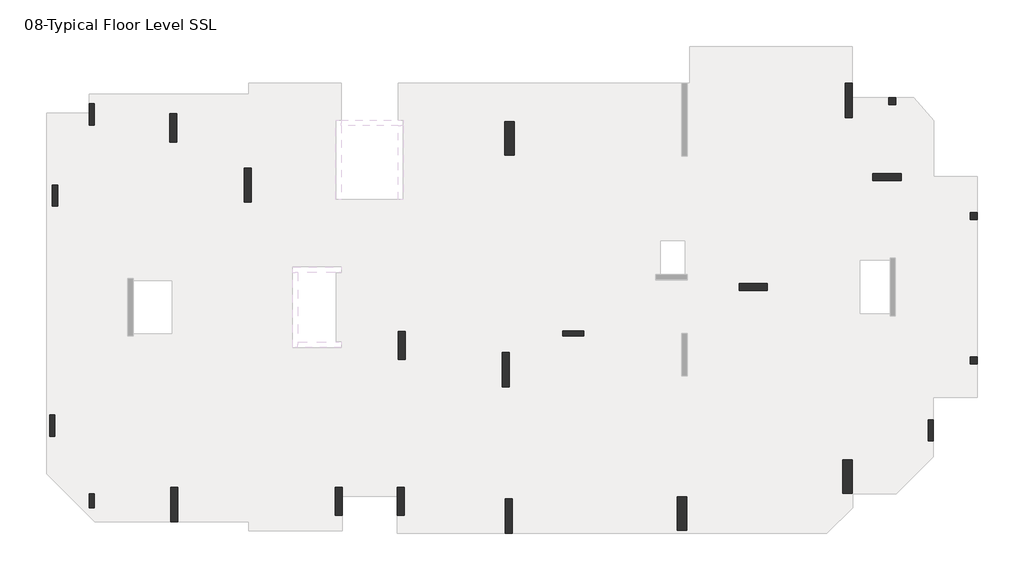
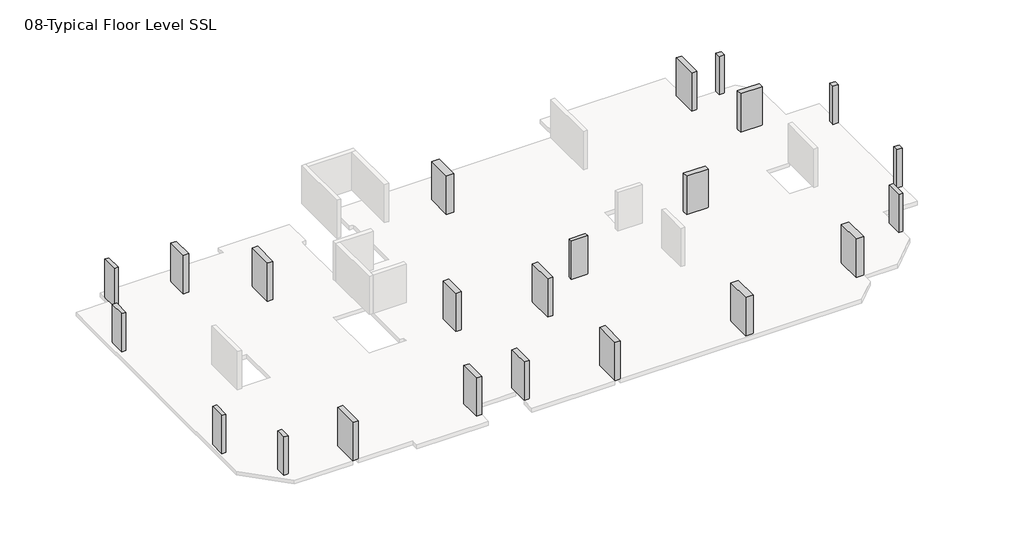
# One storey, part 2 of 2: 23 columns.
"""IFC4 building model written with IfcOpenShell, lengths in millimetres."""

from ifc_helpers import new_model, si_unit, origin, place, context, project, spatial, faceted_brep, element, save

model = new_model("IFC4")

# Units and contexts
model_context = context("Model", 3, world=origin())
ifc_project = project(units=[si_unit("LENGTHUNIT", "METRE", prefix="MILLI")], contexts=[model_context])

# Site, building, storey
site = spatial("IfcSite", under=ifc_project)
building = spatial("IfcBuilding", under=site)
storey = spatial("IfcBuildingStorey", under=building, Name="08-Typical Floor Level SSL", Elevation=18000.0)

# Columns
placement = place(None, origin())
element("IfcColumn", 1, ObjectType="M_Concrete-Rectangular-Column : C-1 (400 x 400mm)", at=placement, inside=storey, context=model_context, shape_type="Brep", body=[
    faceted_brep([(52549.9999998, 16712.0, 18000.0), (52549.9999998, 16312.0, 18000.0), (52149.9999998, 16312.0, 18000.0), (52149.9999998, 16712.0, 18000.0), (52549.9999998, 16712.0, 21000.0), (52549.9999998, 16312.0, 21000.0), (52549.9999998, 16312.0, 20700.0), (52549.9999998, 16712.0, 20700.0), (52149.9999998, 16312.0, 21000.0), (52149.9999998, 16312.0, 20700.0), (52149.9999998, 16712.0, 21000.0), (52149.9999998, 16712.0, 20700.0)], [[[0, 1, 2, 3]], [[4, 5, 6, 1, 0, 7]], [[5, 8, 9, 2, 1, 6]], [[8, 10, 11, 3, 2, 9]], [[10, 4, 7, 0, 3, 11]], [[4, 10, 8, 5]]]),
])
element("IfcColumn", 2, ObjectType="M_Concrete-Rectangular-Column : C-1 (400 x 400mm)", at=placement, inside=storey, context=model_context, shape_type="Brep", body=[
    faceted_brep([(47898.6337868, 23252.0, 18000.0), (47898.6337868, 22852.0, 18000.0), (47498.6337868, 22852.0, 18000.0), (47498.6337868, 23252.0, 18000.0), (47898.6337868, 23252.0, 21000.0), (47898.6337868, 22852.0, 21000.0), (47898.6337868, 22852.0, 20700.0), (47498.6337868, 22852.0, 21000.0), (47498.6337868, 22852.0, 20700.0), (47498.6337868, 23252.0, 21000.0)], [[[0, 1, 2, 3]], [[4, 5, 6, 1, 0]], [[5, 7, 8, 2, 1, 6]], [[7, 9, 3, 2, 8]], [[9, 4, 0, 3]], [[4, 9, 7, 5]]]),
])
element("IfcColumn", 3, ObjectType="M_Concrete-Rectangular-Column : C-1 (400 x 400mm)", at=placement, inside=storey, context=model_context, shape_type="Brep", body=[
    faceted_brep([(52549.9999998, 8504.0039609, 18000.0), (52549.9999998, 8104.0039609, 18000.0), (52149.9999998, 8104.0039609, 18000.0), (52149.9999998, 8504.0039609, 18000.0), (52549.9999998, 8504.0039609, 21000.0), (52549.9999998, 8104.0039609, 21000.0), (52549.9999998, 8104.0039609, 20700.0), (52549.9999998, 8504.0039609, 20700.0), (52149.9999998, 8104.0039609, 21000.0), (52149.9999998, 8104.0039609, 20700.0), (52149.9999998, 8504.0039609, 21000.0), (52149.9999998, 8504.0039609, 20700.0)], [[[0, 1, 2, 3]], [[4, 5, 6, 1, 0, 7]], [[5, 8, 9, 2, 1, 6]], [[8, 10, 11, 3, 2, 9]], [[10, 4, 7, 0, 3, 11]], [[4, 10, 8, 5]]]),
])
element("IfcColumn", 4, ObjectType="M_Concrete-Rectangular-Column : C-2 (300 x 800mm)", at=placement, inside=storey, context=model_context, shape_type="Brep", body=[
    faceted_brep([(2352.0, 728.0, 18000.0), (2352.0, -72.0, 18000.0), (2052.0, -72.0, 18000.0), (2052.0, 728.0, 18000.0), (2352.0, 728.0, 21000.0), (2352.0, -72.0, 21000.0), (2352.0, -72.0, 20700.0), (2352.0, 728.0, 20700.0), (2052.0, -72.0, 21000.0), (2052.0, -72.0, 20700.0), (2052.0, 728.0, 21000.0), (2052.0, 728.0, 20700.0)], [[[0, 1, 2, 3]], [[4, 5, 6, 1, 0, 7]], [[5, 8, 9, 2, 1, 6]], [[8, 10, 11, 3, 2, 9]], [[10, 4, 7, 0, 3, 11]], [[4, 10, 8, 5]]]),
])
element("IfcColumn", 5, ObjectType="M_Concrete-Rectangular-Column : C-3(300 x 1200mm)", at=placement, inside=storey, context=model_context, shape_type="Brep", body=[
    faceted_brep([(2352.0, 22908.0000656, 18000.0), (2352.0, 21708.0000656, 18000.0), (2052.0, 21708.0000656, 18000.0), (2052.0, 22908.0000656, 18000.0), (2352.0, 22908.0000656, 21000.0), (2352.0, 21708.0000656, 21000.0), (2352.0, 21708.0000656, 20700.0), (2352.0, 22908.0000656, 20700.0), (2052.0, 21708.0000656, 21000.0), (2052.0, 21708.0000656, 20700.0), (2052.0, 22380.0004589, 21000.0), (2052.0, 22908.0000656, 21000.0), (2052.0, 22908.0000656, 20700.0)], [[[0, 1, 2, 3]], [[4, 5, 6, 1, 0, 7]], [[5, 8, 9, 2, 1, 6]], [[8, 10, 11, 12, 3, 2, 9]], [[11, 4, 7, 0, 3, 12]], [[4, 11, 10, 8, 5]]]),
])
element("IfcColumn", 6, ObjectType="M_Concrete-Rectangular-Column : C-3(300 x 1200mm)", at=placement, inside=storey, context=model_context, shape_type="Brep", body=[
    faceted_brep([(257.9999999, 18288.0, 18000.0), (257.9999999, 17088.0, 18000.0), (-42.0000001, 17088.0, 18000.0), (-42.0000001, 18288.0, 18000.0), (257.9999999, 18288.0, 21000.0), (257.9999999, 17088.0, 21000.0), (257.9999999, 17088.0, 20700.0), (257.9999999, 18288.0, 20700.0), (-42.0000001, 17088.0, 21000.0), (-42.0000001, 17088.0, 20700.0), (-42.0000001, 18288.0, 21000.0), (-42.0000001, 18288.0, 20700.0)], [[[0, 1, 2, 3]], [[4, 5, 6, 1, 0, 7]], [[5, 8, 9, 2, 1, 6]], [[8, 10, 11, 3, 2, 9]], [[10, 4, 7, 0, 3, 11]], [[4, 10, 8, 5]]]),
])
element("IfcColumn", 7, ObjectType="M_Concrete-Rectangular-Column : C-3(300 x 1200mm)", at=placement, inside=storey, context=model_context, shape_type="Brep", body=[
    faceted_brep([(108.001803, 5201.9999858, 18000.0), (108.001803, 4001.9999858, 18000.0), (-191.998197, 4001.9999858, 18000.0), (-191.998197, 5201.9999858, 18000.0), (108.001803, 5201.9999858, 21000.0), (108.001803, 4001.9999858, 21000.0), (108.001803, 4001.9999858, 20700.0), (108.001803, 5201.9999858, 20700.0), (-191.998197, 4001.9999858, 21000.0), (-191.998197, 4001.9999858, 20700.0), (-191.998197, 5201.9999858, 21000.0), (-191.998197, 5201.9999858, 20700.0)], [[[0, 1, 2, 3]], [[4, 5, 6, 1, 0, 7]], [[5, 8, 9, 2, 1, 6]], [[8, 10, 11, 3, 2, 9]], [[10, 4, 7, 0, 3, 11]], [[4, 10, 8, 5]]]),
])
element("IfcColumn", 8, ObjectType="M_Concrete-Rectangular-Column : C-3(300 x 1200mm)", at=placement, inside=storey, context=model_context, shape_type="Brep", body=[
    faceted_brep([(50046.0009271, 4931.9999929, 18000.0), (50046.0009271, 3731.9999929, 18000.0), (49746.0009271, 3731.9999929, 18000.0), (49746.0009271, 4931.9999929, 18000.0), (50046.0009271, 4931.9999929, 21000.0), (50046.0009271, 3731.9999929, 21000.0), (50046.0009271, 3731.9999929, 20700.0), (50046.0009271, 4931.9999929, 20700.0), (49746.0009271, 3731.9999929, 21000.0), (49746.0009271, 3731.9999929, 20700.0), (49746.0009271, 4931.9999929, 21000.0), (49746.0009271, 4931.9999929, 20700.0)], [[[0, 1, 2, 3]], [[4, 5, 6, 1, 0, 7]], [[5, 8, 9, 2, 1, 6]], [[8, 10, 11, 3, 2, 9]], [[10, 4, 7, 0, 3, 11]], [[4, 10, 8, 5]]]),
])
element("IfcColumn", 9, ObjectType="M_Concrete-Rectangular-Column : C-3(300 x 1200mm)", at=placement, inside=storey, context=model_context, shape_type="Brep", body=[
    faceted_brep([(28975.9999998, 9996.0000019, 18000.0), (30175.9999998, 9996.0000019, 18000.0), (30175.9999998, 9696.0000019, 18000.0), (28975.9999998, 9696.0000019, 18000.0), (28975.9999998, 9996.0000019, 21000.0), (30175.9999998, 9996.0000019, 21000.0), (30175.9999998, 9996.0000019, 20700.0), (28975.9999998, 9996.0000019, 20700.0), (30175.9999998, 9696.0000019, 21000.0), (30175.9999998, 9696.0000019, 20700.0), (28975.9999998, 9696.0000019, 21000.0), (28975.9999998, 9696.0000019, 20700.0)], [[[0, 1, 2, 3]], [[4, 5, 6, 1, 0, 7]], [[5, 8, 9, 2, 1, 6]], [[8, 10, 11, 3, 2, 9]], [[10, 4, 7, 0, 3, 11]], [[4, 10, 8, 5]]]),
])
element("IfcColumn", 10, ObjectType="M_Concrete-Rectangular-Column : C-4 (400 x 1600mm)", at=placement, inside=storey, context=model_context, shape_type="Brep", body=[
    faceted_brep([(7021.9999999, 22340.0000078, 18000.0), (7021.9999999, 20740.0000078, 18000.0), (6621.9999999, 20740.0000078, 18000.0), (6621.9999999, 22340.0000078, 18000.0), (7021.9999999, 22340.0000078, 21000.0), (7021.9999999, 20740.0000078, 21000.0), (7021.9999999, 20740.0000078, 20700.0), (7021.9999999, 22340.0000078, 20700.0), (6621.9999999, 20740.0000078, 21000.0), (6621.9999999, 20740.0000078, 20700.0), (6621.9999999, 22340.0000078, 21000.0), (6621.9999999, 22340.0000078, 20700.0)], [[[0, 1, 2, 3]], [[4, 5, 6, 1, 0, 7]], [[5, 8, 9, 2, 1, 6]], [[8, 10, 11, 3, 2, 9]], [[10, 4, 7, 0, 3, 11]], [[4, 10, 8, 5]]]),
])
element("IfcColumn", 11, ObjectType="M_Concrete-Rectangular-Column : C-4 (400 x 1600mm)", at=placement, inside=storey, context=model_context, shape_type="Brep", body=[
    faceted_brep([(19969.9997488, 1087.9955348, 18000.0), (19969.9997488, -512.0044652, 18000.0), (19569.9997488, -512.0044652, 18000.0), (19569.9997488, 1087.9955348, 18000.0), (19969.9997488, 1087.9955348, 21000.0), (19969.9997488, -512.0044652, 21000.0), (19969.9997488, -512.0044652, 20700.0), (19969.9997488, 1087.9955348, 20700.0), (19569.9997488, -512.0044652, 21000.0), (19569.9997488, -512.0044652, 20700.0), (19569.9997488, 564.000519, 21000.0), (19569.9997488, 1087.9955348, 21000.0), (19569.9997488, 1087.9955348, 20700.0)], [[[0, 1, 2, 3]], [[4, 5, 6, 1, 0, 7]], [[5, 8, 9, 2, 1, 6]], [[8, 10, 11, 12, 3, 2, 9]], [[11, 4, 7, 0, 3, 12]], [[4, 11, 10, 8, 5]]]),
])
element("IfcColumn", 12, ObjectType="M_Concrete-Rectangular-Column : C-4 (400 x 1600mm)", at=placement, inside=storey, context=model_context, shape_type="Brep", body=[
    faceted_brep([(46605.9993605, 18950.0, 18000.0), (48205.9993605, 18950.0, 18000.0), (48205.9993605, 18550.0, 18000.0), (46605.9993605, 18550.0, 18000.0), (46605.9993605, 18950.0, 21000.0), (48205.9993605, 18950.0, 21000.0), (48205.9993605, 18950.0, 20700.0), (46605.9993605, 18950.0, 20700.0), (48205.9993605, 18550.0, 21000.0), (48205.9993605, 18550.0, 20700.0), (46605.9993605, 18550.0, 21000.0), (46605.9993605, 18550.0, 20700.0)], [[[0, 1, 2, 3]], [[4, 5, 6, 1, 0, 7]], [[5, 8, 9, 2, 1, 6]], [[8, 10, 11, 3, 2, 9]], [[10, 4, 7, 0, 3, 11]], [[4, 10, 8, 5]]]),
])
element("IfcColumn", 13, ObjectType="M_Concrete-Rectangular-Column : C-5 (400 x 1600mm)", at=placement, inside=storey, context=model_context, shape_type="Brep", body=[
    faceted_brep([(20030.000009, 9955.9999979, 18000.0), (20030.000009, 8355.9999979, 18000.0), (19630.000009, 8355.9999979, 18000.0), (19630.000009, 9955.9999979, 18000.0), (20030.000009, 9955.9999979, 21000.0), (20030.000009, 8355.9999979, 21000.0), (20030.000009, 8355.9999979, 20700.0), (20030.000009, 9955.9999979, 20700.0), (19630.000009, 8355.9999979, 21000.0), (19630.000009, 8355.9999979, 20700.0), (19630.000009, 9955.9999979, 21000.0), (19630.000009, 9955.9999979, 20700.0)], [[[0, 1, 2, 3]], [[4, 5, 6, 1, 0, 7]], [[5, 8, 9, 2, 1, 6]], [[8, 10, 11, 3, 2, 9]], [[10, 4, 7, 0, 3, 11]], [[4, 10, 8, 5]]]),
])
element("IfcColumn", 14, ObjectType="M_Concrete-Rectangular-Column : C-5 (400 x 1600mm)", at=placement, inside=storey, context=model_context, shape_type="Brep", body=[
    faceted_brep([(16429.9999981, 1088.0, 18000.0), (16429.9999981, -512.0, 18000.0), (16029.9999981, -512.0, 18000.0), (16029.9999981, 1088.0, 18000.0), (16429.9999981, 1088.0, 21000.0), (16429.9999981, 564.000519, 21000.0), (16429.9999981, -512.0, 21000.0), (16429.9999981, -512.0, 20700.0), (16429.9999981, 1088.0, 20700.0), (16029.9999981, -512.0, 21000.0), (16029.9999981, -512.0, 20700.0), (16029.9999981, 1088.0, 21000.0), (16029.9999981, 1088.0, 20700.0)], [[[0, 1, 2, 3]], [[4, 5, 6, 7, 1, 0, 8]], [[6, 9, 10, 2, 1, 7]], [[9, 11, 12, 3, 2, 10]], [[11, 4, 8, 0, 3, 12]], [[4, 11, 9, 6, 5]]]),
])
element("IfcColumn", 15, ObjectType="M_Concrete-Rectangular-Column : C-5 (400 x 1600mm)", at=placement, inside=storey, context=model_context, shape_type="Brep", body=[
    faceted_brep([(38998.0014887, 12692.0079212, 18000.0), (40598.0014887, 12692.0079212, 18000.0), (40598.0014887, 12292.0079212, 18000.0), (38998.0014887, 12292.0079212, 18000.0), (38998.0014887, 12692.0079212, 21000.0), (40598.0014887, 12692.0079212, 21000.0), (40598.0014887, 12692.0079212, 20700.0), (38998.0014887, 12692.0079212, 20700.0), (40598.0014887, 12292.0079212, 21000.0), (40598.0014887, 12292.0079212, 20700.0), (38998.0014887, 12292.0079212, 21000.0), (38998.0014887, 12292.0079212, 20700.0)], [[[0, 1, 2, 3]], [[4, 5, 6, 1, 0, 7]], [[5, 8, 9, 2, 1, 6]], [[8, 10, 11, 3, 2, 9]], [[10, 4, 7, 0, 3, 11]], [[4, 10, 8, 5]]]),
])
element("IfcColumn", 16, ObjectType="M_Concrete-Rectangular-Column : C-6 (400 x 1950mm)", at=placement, inside=storey, context=model_context, shape_type="Brep", body=[
    faceted_brep([(11270.0000427, 19262.9999996, 18000.0), (11270.0000427, 17312.9999996, 18000.0), (10870.0000427, 17312.9999996, 18000.0), (10870.0000427, 19262.9999996, 18000.0), (11270.0000427, 19262.9999996, 21000.0), (11270.0000427, 17312.9999996, 21000.0), (11270.0000427, 17312.9999996, 20700.0), (11270.0000427, 19262.9999996, 20700.0), (10870.0000427, 17312.9999996, 21000.0), (10870.0000427, 17312.9999996, 20700.0), (10870.0000427, 19262.9999996, 21000.0), (10870.0000427, 19262.9999996, 20700.0)], [[[0, 1, 2, 3]], [[4, 5, 6, 1, 0, 7]], [[5, 8, 9, 2, 1, 6]], [[8, 10, 11, 3, 2, 9]], [[10, 4, 7, 0, 3, 11]], [[4, 10, 8, 5]]]),
])
element("IfcColumn", 17, ObjectType="M_Concrete-Rectangular-Column : C-6 (400 x 1950mm)", at=placement, inside=storey, context=model_context, shape_type="Brep", body=[
    faceted_brep([(7082.0000416, 1083.0000153, 18000.0), (7082.0000416, -866.9999847, 18000.0), (6682.0000416, -866.9999847, 18000.0), (6682.0000416, 1083.0000153, 18000.0), (7082.0000416, 1083.0000153, 21000.0), (7082.0000416, -866.9999847, 21000.0), (7082.0000416, -866.9999847, 20700.0), (7082.0000416, 1083.0000153, 20700.0), (6682.0000416, -866.9999847, 21000.0), (6682.0000416, -866.9999847, 20700.0), (6682.0000416, 1083.0000153, 21000.0), (6682.0000416, 1083.0000153, 20700.0)], [[[0, 1, 2, 3]], [[4, 5, 6, 1, 0, 7]], [[5, 8, 9, 2, 1, 6]], [[8, 10, 11, 3, 2, 9]], [[10, 4, 7, 0, 3, 11]], [[4, 10, 8, 5]]]),
])
element("IfcColumn", 18, ObjectType="M_Concrete-Rectangular-Column : C-6 (400 x 1950mm)", at=placement, inside=storey, context=model_context, shape_type="Brep", body=[
    faceted_brep([(26113.9999998, 422.995535, 18000.0), (26113.9999998, -1527.004465, 18000.0), (25713.9999998, -1527.004465, 18000.0), (25713.9999998, 422.995535, 18000.0), (26113.9999998, 422.995535, 21000.0), (26113.9999998, -1527.004465, 21000.0), (26113.9999998, -1527.004465, 20700.0), (26113.9999998, 422.995535, 20700.0), (25713.9999998, -1527.004465, 21000.0), (25713.9999998, -1527.004465, 20700.0), (25713.9999998, 422.995535, 21000.0), (25713.9999998, 422.995535, 20700.0)], [[[0, 1, 2, 3]], [[4, 5, 6, 1, 0, 7]], [[5, 8, 9, 2, 1, 6]], [[8, 10, 11, 3, 2, 9]], [[10, 4, 7, 0, 3, 11]], [[4, 10, 8, 5]]]),
])
element("IfcColumn", 19, ObjectType="M_Concrete-Rectangular-Column : C-6 (400 x 1950mm)", at=placement, inside=storey, context=model_context, shape_type="Brep", body=[
    faceted_brep([(45446.0007483, 24087.0, 18000.0), (45446.0007483, 22137.0, 18000.0), (45046.0007483, 22137.0, 18000.0), (45046.0007483, 24087.0, 18000.0), (45446.0007483, 24087.0, 21000.0), (45446.0007483, 23252.0000315, 21000.0), (45446.0007483, 22137.0, 21000.0), (45446.0007483, 22137.0, 20700.0), (45446.0007483, 24087.0, 20700.0), (45046.0007483, 22137.0, 21000.0), (45046.0007483, 22137.0, 20700.0), (45046.0007483, 24087.0, 21000.0), (45046.0007483, 24087.0, 20700.0)], [[[0, 1, 2, 3]], [[4, 5, 6, 7, 1, 0, 8]], [[6, 9, 10, 2, 1, 7]], [[9, 11, 12, 3, 2, 10]], [[11, 4, 8, 0, 3, 12]], [[4, 11, 9, 6, 5]]]),
])
element("IfcColumn", 20, ObjectType="M_Concrete-Rectangular-Column : C-6 (400 x 1950mm)", at=placement, inside=storey, context=model_context, shape_type="Brep", body=[
    faceted_brep([(25934.0000455, 8751.0001824, 18000.0), (25934.0000455, 6801.0001824, 18000.0), (25534.0000455, 6801.0001824, 18000.0), (25534.0000455, 8751.0001824, 18000.0), (25934.0000455, 8751.0001824, 21000.0), (25934.0000455, 6801.0001824, 21000.0), (25934.0000455, 6801.0001824, 20700.0), (25934.0000455, 8751.0001824, 20700.0), (25534.0000455, 6801.0001824, 21000.0), (25534.0000455, 6801.0001824, 20700.0), (25534.0000455, 8751.0001824, 21000.0), (25534.0000455, 8751.0001824, 20700.0)], [[[0, 1, 2, 3]], [[4, 5, 6, 1, 0, 7]], [[5, 8, 9, 2, 1, 6]], [[8, 10, 11, 3, 2, 9]], [[10, 4, 7, 0, 3, 11]], [[4, 10, 8, 5]]]),
])
element("IfcColumn", 21, ObjectType="M_Concrete-Rectangular-Column : C-7 (550 x 1900mm)", at=placement, inside=storey, context=model_context, shape_type="Brep", body=[
    faceted_brep([(36035.9999998, 548.0007983, 18000.0), (36035.9999998, -1351.9992017, 18000.0), (35485.9999998, -1351.9992017, 18000.0), (35485.9999998, 548.0007983, 18000.0), (36035.9999998, 548.0007983, 21000.0), (36035.9999998, -1351.9992017, 21000.0), (36035.9999998, -1351.9992017, 20700.0), (36035.9999998, 548.0007983, 20700.0), (35485.9999998, -1351.9992017, 21000.0), (35485.9999998, -1351.9992017, 20700.0), (35485.9999998, 548.0007983, 21000.0), (35485.9999998, 548.0007983, 20700.0)], [[[0, 1, 2, 3]], [[4, 5, 6, 1, 0, 7]], [[5, 8, 9, 2, 1, 6]], [[8, 10, 11, 3, 2, 9]], [[10, 4, 7, 0, 3, 11]], [[4, 10, 8, 5]]]),
])
element("IfcColumn", 22, ObjectType="M_Concrete-Rectangular-Column : C-7 (550 x 1900mm)", at=placement, inside=storey, context=model_context, shape_type="Brep", body=[
    faceted_brep([(45443.9999998, 2648.0, 18000.0), (45443.9999998, 748.0, 18000.0), (44893.9999998, 748.0, 18000.0), (44893.9999998, 2648.0, 18000.0), (45443.9999998, 2648.0, 21000.0), (45443.9999998, 748.0, 21000.0), (45443.9999998, 748.0, 20700.0), (45443.9999998, 2648.0, 20700.0), (44893.9999998, 748.0, 21000.0), (44893.9999998, 748.0, 20700.0), (44893.9999998, 2648.0, 21000.0), (44893.9999998, 2648.0, 20700.0)], [[[0, 1, 2, 3]], [[4, 5, 6, 1, 0, 7]], [[5, 8, 9, 2, 1, 6]], [[8, 10, 11, 3, 2, 9]], [[10, 4, 7, 0, 3, 11]], [[4, 10, 8, 5]]]),
])
element("IfcColumn", 23, ObjectType="M_Concrete-Rectangular-Column : C-7 (550 x 1900mm)", at=placement, inside=storey, context=model_context, shape_type="Brep", body=[
    faceted_brep([(26218.9999998, 21900.0, 18000.0), (26218.9999998, 20000.0, 18000.0), (25668.9999998, 20000.0, 18000.0), (25668.9999998, 21900.0, 18000.0), (26218.9999998, 21900.0, 21000.0), (26218.9999998, 20000.0, 21000.0), (26218.9999998, 20000.0, 20700.0), (26218.9999998, 21900.0, 20700.0), (25668.9999998, 20000.0, 21000.0), (25668.9999998, 20000.0, 20700.0), (25668.9999998, 21900.0, 21000.0), (25668.9999998, 21900.0, 20700.0)], [[[0, 1, 2, 3]], [[4, 5, 6, 1, 0, 7]], [[5, 8, 9, 2, 1, 6]], [[8, 10, 11, 3, 2, 9]], [[10, 4, 7, 0, 3, 11]], [[4, 10, 8, 5]]]),
])

save(model, "model.ifc")

# Revit data of these elements
# Type "M_Concrete-Rectangular-Column : C-1 (400 x 400mm)"
#   Type Mark = "C01"
#   b = 400 mm
#   h = 400 mm
#   Structural Material [instance default] = Concrete, Cast-in-Place gray
# Type "M_Concrete-Rectangular-Column : C-2 (300 x 800mm)"
#   Type Mark = "C02"
#   b = 300 mm
#   h = 800 mm
#   Structural Material [instance default] = Concrete, Cast-in-Place gray
# Type "M_Concrete-Rectangular-Column : C-3(300 x 1200mm)"
#   Type Mark = "C03"
#   b = 300 mm
#   h = 1200 mm
#   Structural Material [instance default] = Concrete, Cast-in-Place gray
# Type "M_Concrete-Rectangular-Column : C-4 (400 x 1600mm)"
#   Type Mark = "C04"
#   b = 400 mm
#   h = 1600 mm
#   Structural Material [instance default] = Concrete, Cast-in-Place gray
# Type "M_Concrete-Rectangular-Column : C-5 (400 x 1600mm)"
#   Type Mark = "C05"
#   b = 400 mm
#   h = 1600 mm
#   Structural Material [instance default] = Concrete, Cast-in-Place gray
# Type "M_Concrete-Rectangular-Column : C-6 (400 x 1950mm)"
#   Type Mark = "C06"
#   b = 400 mm
#   h = 1950 mm
#   Structural Material [instance default] = Concrete, Cast-in-Place gray
# Type "M_Concrete-Rectangular-Column : C-7 (550 x 1900mm)"
#   Type Mark = "C07"
#   b = 550 mm
#   h = 1900 mm
#   Structural Material [instance default] = Concrete, Cast-in-Place gray
# Elements 1, 2, 3 (IfcColumn, "M_Concrete-Rectangular-Column : C-1 (400 x 400mm)")
#   Structural Material = Concrete-RC
#   Phase Created = New Construction
#   Materials on its faces: "Concrete-RC"
# Element 4 (IfcColumn, "M_Concrete-Rectangular-Column : C-2 (300 x 800mm)")
#   Structural Material = Concrete-RC
#   Phase Created = New Construction
#   Materials on its faces: "Concrete-RC"
# Elements 5, 6, 7, 8, 9 (IfcColumn, "M_Concrete-Rectangular-Column : C-3(300 x 1200mm)")
#   Structural Material = Concrete-RC
#   Phase Created = New Construction
#   Materials on its faces: "Concrete-RC"
# Elements 10, 11, 12 (IfcColumn, "M_Concrete-Rectangular-Column : C-4 (400 x 1600mm)")
#   Structural Material = Concrete-RC
#   Phase Created = New Construction
#   Materials on its faces: "Concrete-RC"
# Elements 13, 14, 15 (IfcColumn, "M_Concrete-Rectangular-Column : C-5 (400 x 1600mm)")
#   Structural Material = Concrete-RC
#   Phase Created = New Construction
#   Materials on its faces: "Concrete-RC"
# Elements 16, 17, 18, 19, 20 (IfcColumn, "M_Concrete-Rectangular-Column : C-6 (400 x 1950mm)")
#   Structural Material = Concrete-RC
#   Phase Created = New Construction
#   Materials on its faces: "Concrete-RC"
# Elements 21, 22, 23 (IfcColumn, "M_Concrete-Rectangular-Column : C-7 (550 x 1900mm)")
#   Structural Material = Concrete-RC
#   Phase Created = New Construction
#   Materials on its faces: "Concrete-RC"
# Materials
#   "Concrete, Cast-in-Place gray": class "Concrete", colour RGB 192 192 192, transparency 0, Description = "Cast-in-place concrete", Cost = 0
#   "Concrete-RC": class "Concrete", colour RGB 128 128 128, transparency 0, Description = "High strength concrete", Cost = 0
